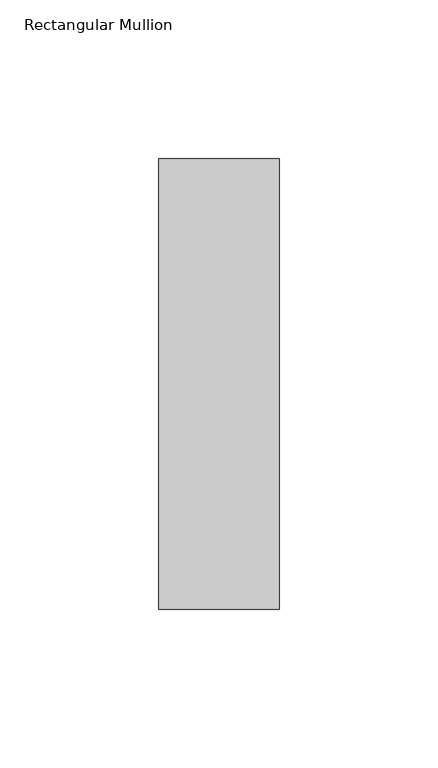
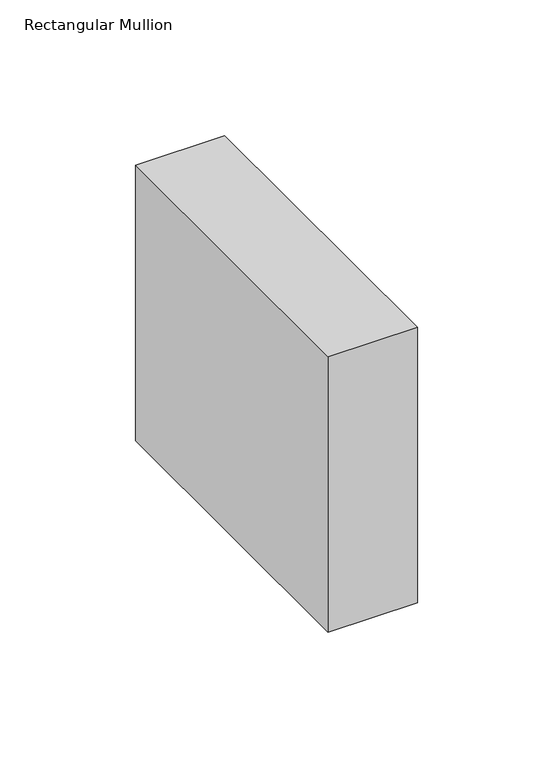
"""IFC4 building model written with IfcOpenShell, lengths in millimetres: member geometry, Rectangular Mullion : NLRS_21_CWM_hsb-regel 38x142_gen_rsf."""

from ifc_helpers import new_model, si_unit, frame, origin, place, context, project, spatial, polyline, outline, extrude, source, transform, mapped, element, save


def rectangular_mullion_0b08a0e2(model_context):
    return source(origin(), model_context, "Body", "SweptSolid", [
        extrude(outline(polyline([(0.0, -71.0), (-38.0, -71.0), (-38.0, 71.0), (0.0, 71.0), (0.0, -71.0)])), frame((0.0, 0.0, -123.9999997), z_axis=(0.0, 0.0, 1.0), x_axis=(1.0, 0.0, 0.0)), (0.0, 0.0, 1.0), 123.9999997),
    ])


if __name__ == "__main__":
    model = new_model("IFC4")
    model_context = context("Model", 3, world=origin())
    ifc_project = project(units=[si_unit("LENGTHUNIT", "METRE", prefix="MILLI")], contexts=[model_context])
    site = spatial("IfcSite", under=ifc_project)
    building = spatial("IfcBuilding", under=site)
    placement = place(None, origin())
    rectangular_mullion_shape = rectangular_mullion_0b08a0e2(model_context)
    element("IfcMember", 1, ObjectType="Rectangular Mullion : NLRS_21_CWM_hsb-regel 38x142_gen_rsf", at=placement, inside=building, context=model_context, shape_type="MappedRepresentation", body=[
        mapped(rectangular_mullion_shape, transform((0.0, 0.0, 0.0), x_axis=(1.0, 0.0, 0.0), y_axis=(0.0, 1.0, 0.0), z_axis=(0.0, 0.0, 1.0))),
    ])
    save(model, "model.ifc")

# Revit data of these elements
# Type "Rectangular Mullion : NLRS_21_CWM_hsb-regel 38x142_gen_rsf"
#   Export Type to IFC As = "IfcWall"
#   Type IfcGUID = "07M7mRoiH1CR8m_RSKIwpF"
#   Assembly Code = "21.10"
#   built-in parameter 1007322 = 0.465879 (stored number, unit not read)
#   built-in parameter 1007321 = 0.062336 (stored number, unit not read)
#   built-in parameter 1007320 = 0.062336 (stored number, unit not read)
# Element 1 (IfcMember, "Rectangular Mullion : NLRS_21_CWM_hsb-regel 38x142_gen_rsf")
#   Materials on its faces: "NLRS_i2_hout naaldhout vuren_gen_rsf"
# Materials
#   "NLRS_i2_hout naaldhout vuren_gen_rsf": class "I - Hout", colour RGB 234 199 147, transparency 0, Keynote = "i2", Manufacturer = "Revit Standards Foundation", URL = "www.revitstandards.org", Description = "hout vuren", Cost = 0
